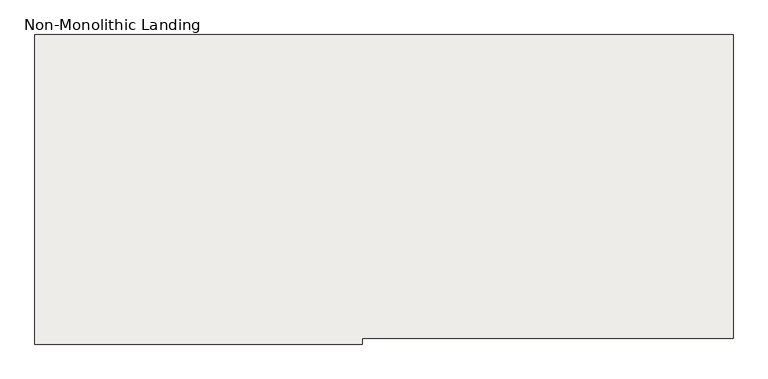
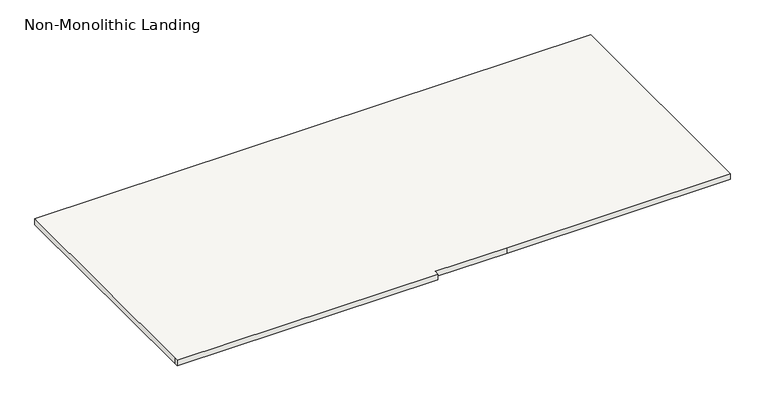
"""IFC4 building model written with IfcOpenShell, lengths in millimetres: slab geometry, Non-Monolithic Landing."""

from ifc_helpers import new_model, si_unit, frame, origin, place, context, project, spatial, polyline, outline, extrude, source, transform, mapped, element, save


def non_monolithic_landing_f0fc5e98(model_context):
    return source(origin(), model_context, "Body", "SweptSolid", [
        extrude(outline(polyline([(-22581.8414763, -9454.4070712), (-22877.1164763, -9454.4070712), (-22877.1164763, -9473.4570712), (-23943.9164763, -9473.4570712), (-23943.9164763, -9454.4070712), (-23943.9164763, -8463.8070712), (-21667.4414763, -8463.8070712), (-21667.4414763, -9454.4070712), (-22581.8414763, -9454.4070712)])), frame((0.0, 0.0, 1318.4782813), z_axis=(0.0, 0.0, 1.0), x_axis=(1.0, 0.0, 0.0)), (0.0, 0.0, 1.0), 23.9117187),
    ])


if __name__ == "__main__":
    model = new_model("IFC4")
    model_context = context("Model", 3, world=origin())
    ifc_project = project(units=[si_unit("LENGTHUNIT", "METRE", prefix="MILLI")], contexts=[model_context])
    site = spatial("IfcSite", under=ifc_project)
    building = spatial("IfcBuilding", under=site)
    placement = place(None, origin())
    non_monolithic_landing_shape = non_monolithic_landing_f0fc5e98(model_context)
    element("IfcSlab", 1, ObjectType="Non-Monolithic Landing", at=placement, inside=building, context=model_context, shape_type="MappedRepresentation", body=[
        mapped(non_monolithic_landing_shape, transform((0.0, 0.0, 0.0), x_axis=(1.0, 0.0, 0.0), y_axis=(0.0, 1.0, 0.0), z_axis=(0.0, 0.0, 1.0))),
    ])
    save(model, "model.ifc")

# Revit data of these elements
# Element 1 (IfcSlab, "Non-Monolithic Landing")
#   Materials on its faces: "DEFAULT DOOR"
# Materials
#   "DEFAULT DOOR": class "Generic", colour RGB 216 216 216, transparency 0, Cost = 0
